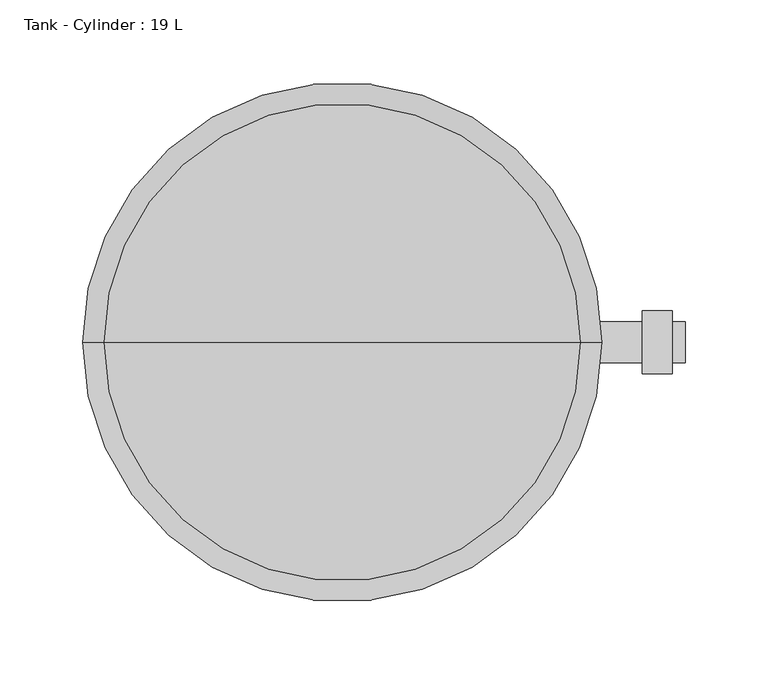
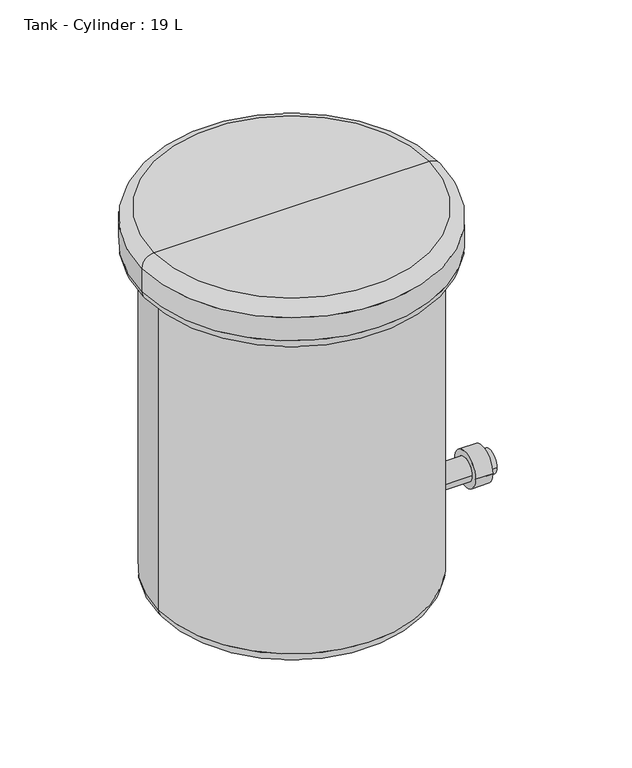
"""IFC4 building model written with IfcOpenShell, lengths in millimetres: proxy geometry, Tank - Cylinder : 19 L."""

from ifc_helpers import new_model, si_unit, point, frame, origin, place, context, project, spatial, circle_curve, ellipse_curve, trimmed, source, transform, mapped, element, save
from ifc_brep_helpers import plane_surface, cylinder_surface, revolved_surface, advanced_brep


def tank_cylinder_19_l_e9b535fb(model_context):
    return source(origin(), model_context, "Body", "AdvancedBrep", [
        advanced_brep(
        [(199.7, -19.0, 56.0), (199.7, 19.0, 56.0), (199.7, 12.5, 56.0), (199.7, -12.5, 56.0), (181.7, -19.0, 56.0), (181.7, 19.0, 56.0), (181.7, -12.5, 56.0), (181.7, 12.5, 56.0), (207.7, -12.5, 56.0), (207.7, 12.5, 56.0), (139.7, -12.5, 56.0), (139.7, 0.0, 68.5), (139.7, 12.5, 56.0), (139.7, 0.0, 43.5)],
        [
            (0, 1, circle_curve(frame((199.7, 0.0, 56.0), z_axis=(1.0, 0.0, 0.0), x_axis=(0.0, 1.0, 0.0)), 19.0)),
            (1, 0, circle_curve(frame((199.7, 0.0, 56.0), z_axis=(1.0, 0.0, 0.0), x_axis=(0.0, 1.0, 0.0)), 19.0)),
            (2, 3, circle_curve(frame((199.7, 0.0, 56.0), z_axis=(-1.0, 0.0, 0.0), x_axis=(0.0, 1.0, 0.0)), 12.5)),
            (3, 2, circle_curve(frame((199.7, 0.0, 56.0), z_axis=(-1.0, 0.0, 0.0), x_axis=(0.0, 1.0, 0.0)), 12.5)),
            (4, 5, circle_curve(frame((181.7, 0.0, 56.0), z_axis=(-1.0, 0.0, 0.0), x_axis=(0.0, 1.0, 0.0)), 19.0)),
            (5, 4, circle_curve(frame((181.7, 0.0, 56.0), z_axis=(-1.0, 0.0, 0.0), x_axis=(0.0, 1.0, 0.0)), 19.0)),
            (6, 7, circle_curve(frame((181.7, 0.0, 56.0), z_axis=(1.0, 0.0, 0.0), x_axis=(0.0, 1.0, 0.0)), 12.5)),
            (7, 6, circle_curve(frame((181.7, 0.0, 56.0), z_axis=(1.0, 0.0, 0.0), x_axis=(0.0, 1.0, 0.0)), 12.5)),
            (0, 4),
            (5, 1),
            (8, 9, circle_curve(frame((207.7, 0.0, 56.0), z_axis=(1.0, 0.0, 0.0), x_axis=(0.0, 1.0, 0.0)), 12.5)),
            (9, 8, circle_curve(frame((207.7, 0.0, 56.0), z_axis=(1.0, 0.0, 0.0), x_axis=(0.0, 1.0, 0.0)), 12.5)),
            (10, 11, circle_curve(frame((139.7, 0.0, 56.0), z_axis=(-1.0, 0.0, 0.0), x_axis=(0.0, 1.0, 0.0)), 12.5)),
            (11, 12, circle_curve(frame((139.7, 0.0, 56.0), z_axis=(-1.0, 0.0, 0.0), x_axis=(0.0, 1.0, 0.0)), 12.5)),
            (12, 13, circle_curve(frame((139.7, 0.0, 56.0), z_axis=(-1.0, 0.0, 0.0), x_axis=(0.0, 1.0, 0.0)), 12.5)),
            (13, 10, circle_curve(frame((139.7, 0.0, 56.0), z_axis=(-1.0, 0.0, 0.0), x_axis=(0.0, 1.0, 0.0)), 12.5)),
            (8, 3),
            (2, 9),
            (6, 10),
            (12, 7),
        ],
        [
            plane_surface(frame((199.7, 19.0, 56.0), z_axis=(1.0, 0.0, 0.0), x_axis=(0.0, 0.0, 1.0))),
            plane_surface(frame((181.7, 19.0, 56.0), z_axis=(-1.0, 0.0, 0.0), x_axis=(0.0, 0.0, -1.0))),
            cylinder_surface(frame((181.7, 0.0, 56.0), z_axis=(1.0, 0.0, 0.0), x_axis=(0.0, 1.0, 0.0)), 19.0),
            plane_surface(frame((207.7, 12.5, 56.0), z_axis=(1.0, 0.0, 0.0), x_axis=(0.0, 0.0, 1.0))),
            plane_surface(frame((139.7, 12.5, 56.0), z_axis=(-1.0, 0.0, 0.0), x_axis=(0.0, 0.0, -1.0))),
            cylinder_surface(frame((139.7, 0.0, 56.0), z_axis=(1.0, 0.0, 0.0), x_axis=(0.0, 1.0, 0.0)), 12.5),
        ],
        [
            (0, [[1, 2], [3, 4]]),
            (1, [[5, 6], [7, 8]]),
            (2, [[-1, 9, -6, 10]]),
            (2, [[-2, -10, -5, -9]]),
            (3, [[11, 12]]),
            (4, [[13, 14, 15, 16]]),
            (5, [[-11, 17, -3, 18]]),
            (5, [[19, -16, -15, 20, -7]]),
            (5, [[-12, -18, -4, -17]]),
            (5, [[-19, -8, -20, -14, -13]]),
        ],
    ),
        advanced_brep(
        [(157.15, 0.0, 396.9), (-157.15, 0.0, 396.9), (-144.45, 0.0, 409.6), (144.45, 0.0, 409.6), (157.15, 0.0, 371.5), (-157.15, 0.0, 371.5), (144.45, 0.0, 358.8), (-144.45, 0.0, 358.8), (139.7, 0.0, 358.8), (-139.7, 0.0, 358.8), (139.7, 0.0, 68.5), (139.7, 0.0, 43.5), (139.7, 0.0, 12.7), (-139.7, 0.0, 12.7), (127.0, 0.0, 0.0), (-127.0, 0.0, 0.0), (0.0, 0.0, 0.0), (0.0, 0.0, 409.6)],
        [
            (0, 1, circle_curve(frame((0.0, 0.0, 396.9), z_axis=(0.0, 0.0, 1.0), x_axis=(-1.0, 0.0, 0.0)), 157.15)),
            (1, 2, circle_curve(frame((-144.45, 0.0, 396.9), z_axis=(0.0, 1.0, 0.0), x_axis=(1.0, 0.0, 0.0)), 12.7)),
            (2, 3, circle_curve(frame((0.0, 0.0, 409.6), z_axis=(0.0, 0.0, -1.0), x_axis=(-1.0, 0.0, 0.0)), 144.45)),
            (3, 0, circle_curve(frame((144.45, 0.0, 396.9), z_axis=(0.0, 1.0, 0.0), x_axis=(-1.0, 0.0, 0.0)), 12.7)),
            (1, 0, circle_curve(frame((0.0, 0.0, 396.9), z_axis=(0.0, 0.0, 1.0), x_axis=(-1.0, 0.0, 0.0)), 157.15)),
            (3, 2, circle_curve(frame((0.0, 0.0, 409.6), z_axis=(0.0, 0.0, -1.0), x_axis=(-1.0, 0.0, 0.0)), 144.45)),
            (0, 4),
            (4, 5, circle_curve(frame((0.0, 0.0, 371.5), z_axis=(0.0, 0.0, 1.0), x_axis=(-1.0, 0.0, 0.0)), 157.15)),
            (5, 1),
            (5, 4, circle_curve(frame((0.0, 0.0, 371.5), z_axis=(0.0, 0.0, 1.0), x_axis=(-1.0, 0.0, 0.0)), 157.15)),
            (4, 6, circle_curve(frame((144.45, 0.0, 371.5), z_axis=(0.0, 1.0, 0.0), x_axis=(-1.0, 0.0, 0.0)), 12.7)),
            (6, 7, circle_curve(frame((0.0, 0.0, 358.8), z_axis=(0.0, 0.0, 1.0), x_axis=(-1.0, 0.0, 0.0)), 144.45)),
            (7, 5, circle_curve(frame((-144.45, 0.0, 371.5), z_axis=(0.0, 1.0, 0.0), x_axis=(1.0, 0.0, 0.0)), 12.7)),
            (7, 6, circle_curve(frame((0.0, 0.0, 358.8), z_axis=(0.0, 0.0, 1.0), x_axis=(-1.0, 0.0, 0.0)), 144.45)),
            (6, 8),
            (8, 9, circle_curve(frame((0.0, 0.0, 358.8), z_axis=(0.0, 0.0, 1.0), x_axis=(-1.0, 0.0, 0.0)), 139.7)),
            (9, 7),
            (9, 8, circle_curve(frame((0.0, 0.0, 358.8), z_axis=(0.0, 0.0, 1.0), x_axis=(-1.0, 0.0, 0.0)), 139.7)),
            (8, 10),
            (10, 11),
            (11, 12),
            (12, 13, circle_curve(frame((0.0, 0.0, 12.7), z_axis=(0.0, 0.0, 1.0), x_axis=(-1.0, 0.0, 0.0)), 139.7)),
            (13, 9),
            (13, 12, circle_curve(frame((0.0, 0.0, 12.7), z_axis=(0.0, 0.0, 1.0), x_axis=(-1.0, 0.0, 0.0)), 139.7)),
            (12, 14, circle_curve(frame((127.0, 0.0, 12.7), z_axis=(0.0, 1.0, 0.0), x_axis=(-1.0, 0.0, 0.0)), 12.7)),
            (14, 15, circle_curve(frame((0.0, 0.0, 0.0), z_axis=(0.0, 0.0, 1.0), x_axis=(-1.0, 0.0, 0.0)), 127.0)),
            (15, 13, circle_curve(frame((-127.0, 0.0, 12.7), z_axis=(0.0, 1.0, 0.0), x_axis=(1.0, 0.0, 0.0)), 12.7)),
            (15, 14, circle_curve(frame((0.0, 0.0, 0.0), z_axis=(0.0, 0.0, 1.0), x_axis=(-1.0, 0.0, 0.0)), 127.0)),
            (14, 16),
            (16, 15),
            (2, 17),
            (17, 3),
        ],
        [
            revolved_surface(trimmed(ellipse_curve(frame((-144.45, 0.0, 396.9), z_axis=(0.0, -1.0, 0.0), x_axis=(1.0, 0.0, 0.0)), 12.7, 12.7), [point((-144.45, 0.0, 409.6))], [point((-157.15, 0.0, 396.9))], True, "CARTESIAN"), (0.0, 0.0, 738.4907028), (0.0, 0.0, -1.0)),
            cylinder_surface(frame((0.0, 0.0, 738.4907028), z_axis=(0.0, 0.0, -1.0), x_axis=(-1.0, 0.0, 0.0)), 157.15),
            revolved_surface(trimmed(ellipse_curve(frame((-144.45, 0.0, 371.5), z_axis=(0.0, -1.0, 0.0), x_axis=(1.0, 0.0, 0.0)), 12.7, 12.7), [point((-157.15, 0.0, 371.5))], [point((-144.45, 0.0, 358.8))], True, "CARTESIAN"), (0.0, 0.0, 738.4907028), (0.0, 0.0, -1.0)),
            plane_surface(frame((0.0, 0.0, 358.8), z_axis=(0.0, 0.0, -1.0), x_axis=(-1.0, 0.0, 0.0))),
            cylinder_surface(frame((0.0, 0.0, 738.4907028), z_axis=(0.0, 0.0, -1.0), x_axis=(-1.0, 0.0, 0.0)), 139.7),
            revolved_surface(trimmed(ellipse_curve(frame((-127.0, 0.0, 12.7), z_axis=(0.0, -1.0, 0.0), x_axis=(1.0, 0.0, 0.0)), 12.7, 12.7), [point((-139.7, 0.0, 12.7))], [point((-127.0, 0.0, 0.0))], True, "CARTESIAN"), (0.0, 0.0, 738.4907028), (0.0, 0.0, -1.0)),
            plane_surface(frame((0.0, 0.0, 0.0), z_axis=(0.0, 0.0, -1.0), x_axis=(-1.0, 0.0, 0.0))),
            plane_surface(frame((0.0, 0.0, 409.6), z_axis=(0.0, 0.0, 1.0), x_axis=(-1.0, 0.0, 0.0))),
        ],
        [
            (0, [[1, 2, 3, 4]]),
            (0, [[-2, 5, -4, 6]]),
            (1, [[-1, 7, 8, 9]]),
            (1, [[-5, -9, 10, -7]]),
            (2, [[-8, 11, 12, 13]]),
            (2, [[-10, -13, 14, -11]]),
            (3, [[-12, 15, 16, 17]]),
            (3, [[-14, -17, 18, -15]]),
            (4, [[-16, 19, 20, 21, 22, 23]]),
            (4, [[-18, -23, 24, -21, -20, -19]]),
            (5, [[-22, 25, 26, 27]]),
            (5, [[-24, -27, 28, -25]]),
            (6, [[-26, 29, 30]]),
            (6, [[-28, -30, -29]]),
            (7, [[-3, 31, 32]]),
            (7, [[-6, -32, -31]]),
        ],
    ),
    ])


if __name__ == "__main__":
    model = new_model("IFC4")
    model_context = context("Model", 3, world=origin())
    ifc_project = project(units=[si_unit("LENGTHUNIT", "METRE", prefix="MILLI")], contexts=[model_context])
    site = spatial("IfcSite", under=ifc_project)
    building = spatial("IfcBuilding", under=site)
    placement = place(None, origin())
    tank_cylinder_19_l_shape = tank_cylinder_19_l_e9b535fb(model_context)
    element("IfcBuildingElementProxy", 1, Name="Tank - Cylinder : 19 L", ObjectType="Tank - Cylinder : 19 L", at=placement, inside=building, context=model_context, shape_type="MappedRepresentation", body=[
        mapped(tank_cylinder_19_l_shape, transform((0.0, 0.0, 0.0), x_axis=(1.0, 0.0, 0.0), y_axis=(0.0, 1.0, 0.0), z_axis=(0.0, 0.0, 1.0))),
    ])
    save(model, "model.ifc")

# Revit data of these elements
# Project information
#   Design Option = "Main Model"
#   Classification.Facility.Description = "Mixed-Gender Dormitory"
#   Classification.Facility.Number = "11-16 27 14"
#   COBie.CreatedBy = "info@mma.ie"
#   COBie.CreatedOn = "2017-07-05T03:26:16"
#   COBie.Facility.Category = "11-16 27 14 : Mixed-Gender Dormitory"
#   COBie.Facility.ProjectName = "East Dormitory"
#   COBie.Facility.SiteName = "East Healey Street, Champaign, Illinois ,USA"
#   COBie.Facility.LinearUnits = "Millimeters"
#   COBie.Facility.AreaUnits = "Square Meters"
#   COBie.Facility.VolumeUnits = "Cubic Meters"
#   COBie.Facility.CurrencyUnit = "None"
#   COBie.Facility.AreaMeasurement = "Revit Default Area Calculation Method"
#   COBie.Facility.Description = "One Four Dormitories Project Site on the E,Healey Site"
#   COBie.Facility.ProjectDescription = "A two Story luxury Dormitory"
#   COBie.Facility.SiteDescription = "Four Dormitories Project Site"
#   COBie.Facility.Phase = "60% Design Submission"
#   Project Issue Date = "Issue Date"
#   Project Status = "Final Issue"
#   Client Name = "Prairie Sky Consulting"
#   Project Address = "East Healey Street, \nChampaign\nIllinois\nUSA"
#   Project Name = "Four Dormitory Complex"
#   Project Number = "East Dormitory"
# Type "Tank - Cylinder : 19 L"
#   Type Mark = "Tank-Cylinder"
#   Classification.OmniClass.23.Number = "23-27 29 19"
#   Classification.OmniClass.23.Description = "Tanks"
#   COBie.Type.CreatedBy = "info@mma.ie"
#   COBie.Type.CreatedOn = "2017-07-05T03:26:17"
#   COBie.Type.Name = "Tank-Cylinder"
#   COBie.Type.Category = "23-27 29 19 : Tanks"
#   COBie.Type.Description = "Tank - Cylinder_19 L"
#   COBie.Type.AssetType = "Fixed"
#   COBie.Type.Manufacturer = ""
#   COBie.Type.ModelNumber = ""
#   T.C. Storage = "19L"
#   Keynote = "43 41 16.16.A"
#   Description = "Tank - Cylinder_19 L"
#   COBie.Type.ReplacementCost = 0
#   T.C. Pipe Diameter = 25 mm
#   T.C. Height = 409.6 mm
#   T.C. Diameter = 314.3 mm
#   RadiusConnectorHead = 19 mm
#   Radius 1 = 12.7 mm
#   NominalSizeConnector = 25 mm
#   NominalRadiusConnector = 12.5 mm
#   Half Dim C = 139.7 mm
#   Flow [instance default] = 0.0 L/s
#   Dim D = 25.4 mm
#   Dim C = 279.4 mm
#   Dim B = 384.2 mm
#   Dim A = 314.3 mm
#   COBie.Type = yes
#   Material = Steel, Wrought
#   Default Elevation = 0
# Element 1 (IfcBuildingElementProxy, "Tank - Cylinder : 19 L")
#   Materials on its faces: "Steel, Wrought"
# Materials
#   "Steel, Wrought": class "Metal", colour RGB 120 120 120, transparency 0, Description = "Wrought steel", Cost = 0
